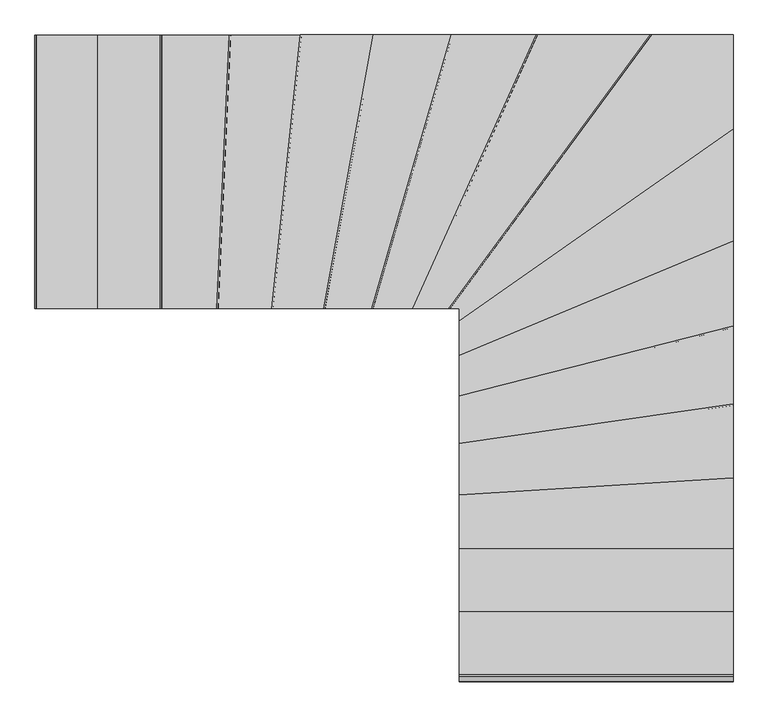
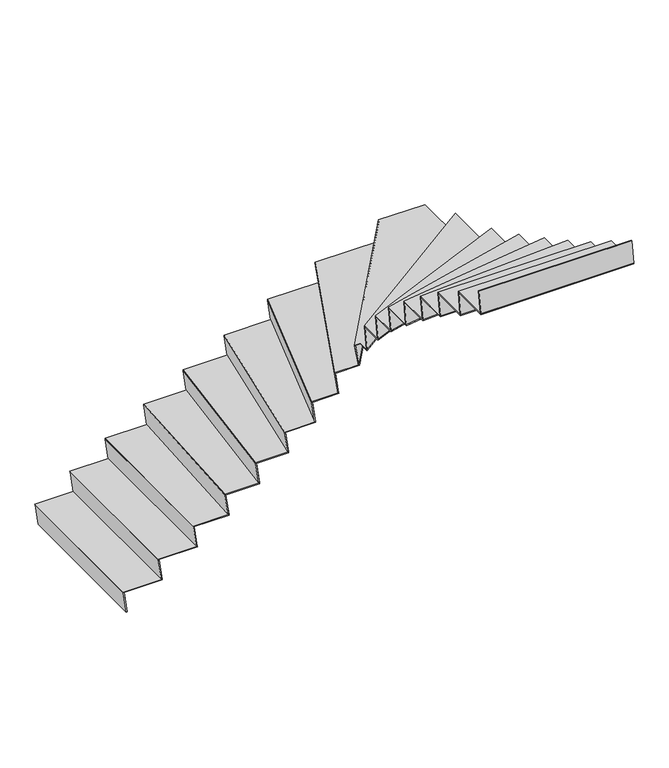
"""IFC4 building model written with IfcOpenShell, lengths in millimetres: stair flight geometry."""

import ifcopenshell
import ifcopenshell.guid

model = None  # the IFC model being written
_history = None  # IfcOwnerHistory: only IFC2X3 demands one
_inside = {}  # id of a spatial element -> (the spatial element, [elements in it])
_under = {}  # id of a project, library or spatial element -> (it, [spatial elements below it])
_declared = {}  # id of a project -> (the project, [libraries it declares])
_typed = {}  # id of a type object -> (the type object, [elements of that type])
_made_of = {}  # id of a material, layer set ... -> (it, [elements and type objects made of it])


def new_model(schema):
    """Start an empty IFC model of exactly this schema.

    Asked for "IFC4X3", IfcOpenShell would pick the latest addendum, in which some entities
    have other attributes; the version numbers below select the first issue.
    IFC2X3 requires an IfcOwnerHistory on every rooted entity: one is made here for all.
    """
    global model, _history
    if schema == "IFC4X3":
        model = ifcopenshell.file(schema_version=(4, 3, 0, 0))
    else:
        model = ifcopenshell.file(schema=schema)
    _inside.clear()
    _under.clear()
    _declared.clear()
    _typed.clear()
    _made_of.clear()
    _history = None
    if model.schema == "IFC2X3":
        org = make("IfcOrganization", Name="unknown")
        user = make(
            "IfcPersonAndOrganization",
            ThePerson=make("IfcPerson", FamilyName="unknown"),
            TheOrganization=org,
        )
        app = make(
            "IfcApplication",
            ApplicationDeveloper=org,
            Version="unknown",
            ApplicationFullName="unknown",
            ApplicationIdentifier="unknown",
        )
        _history = make(
            "IfcOwnerHistory",
            OwningUser=user,
            OwningApplication=app,
            ChangeAction="ADDED",
            CreationDate=0,
        )
    return model


def make(cls, **values):
    """One entity of the class cls with the attributes given. An attribute that is None is left unset."""
    return model.create_entity(
        cls, **{name: value for name, value in values.items() if value is not None}
    )


def rooted(cls, **values):
    """An entity with a GlobalId (a new one), such as an element, a storey or a relation."""
    return make(cls, GlobalId=ifcopenshell.guid.new(), OwnerHistory=_history, **values)


def si_unit(unit_type, name, prefix=None):
    """IfcSIUnit, for example si_unit("LENGTHUNIT", "METRE", prefix="MILLI")."""
    return make("IfcSIUnit", UnitType=unit_type, Prefix=prefix, Name=name)


def assignment(units):
    """IfcUnitAssignment: the units of a project."""
    return None if units is None else make("IfcUnitAssignment", Units=units)


def point(xyz):
    """IfcCartesianPoint."""
    return None if xyz is None else make("IfcCartesianPoint", Coordinates=xyz)


def direction(xyz):
    """IfcDirection."""
    return None if xyz is None else make("IfcDirection", DirectionRatios=xyz)


def frame(location, z_axis=None, x_axis=None):
    """IfcAxis2Placement3D, a coordinate frame: its origin and axes. An axis left out is left unset."""
    return make(
        "IfcAxis2Placement3D",
        Location=point(location),
        Axis=direction(z_axis),
        RefDirection=direction(x_axis),
    )


def origin():
    """The frame at (0, 0, 0) with its axes left unset."""
    return frame((0.0, 0.0, 0.0))


def place(relative_to, where):
    """IfcLocalPlacement: puts the frame where relative to a parent placement (None: the world)."""
    return make(
        "IfcLocalPlacement", PlacementRelTo=relative_to, RelativePlacement=where
    )


def context(
    kind, dimensions, precision=None, world=None, true_north=None, identifier=None
):
    """IfcGeometricRepresentationContext, for example the 3D "Model" context."""
    return make(
        "IfcGeometricRepresentationContext",
        ContextIdentifier=identifier,
        ContextType=kind,
        CoordinateSpaceDimension=dimensions,
        Precision=precision,
        WorldCoordinateSystem=world,
        TrueNorth=true_north,
    )


def project(units=None, contexts=None):
    """IfcProject with its units and contexts."""
    return rooted(
        "IfcProject",
        Name="project",
        RepresentationContexts=contexts,
        UnitsInContext=assignment(units),
    )


def spatial(cls, under=None, at=None, **own):
    """A site, building, storey or space (cls), placed at a placement, below another one or the project."""
    s = rooted(cls, ObjectPlacement=at, **own)
    if under is not None:
        _under.setdefault(under.id(), (under, []))[1].append(s)
    return s


def faces_of(points, faces, orient=None, outer=None):
    """IfcFace entities. A face is a list of loops; a loop is a list of indices into points, from 0.

    orient and outer hold one flag for each loop. By default every Orientation is true, the
    first loop of a face is its IfcFaceOuterBound and the others are IfcFaceBound.
    """
    made = []
    for i, loops in enumerate(faces):
        bounds = []
        for j, loop in enumerate(loops):
            is_outer = j == 0 if outer is None else outer[i][j]
            bounds.append(
                make(
                    "IfcFaceOuterBound" if is_outer else "IfcFaceBound",
                    Bound=make("IfcPolyLoop", Polygon=[points[k] for k in loop]),
                    Orientation=True if orient is None else orient[i][j],
                )
            )
        made.append(make("IfcFace", Bounds=bounds))
    return made


def faceted_brep(points, faces, orient=None, outer=None, voids=None):
    """IfcFacetedBrep: a solid bounded by flat faces; with voids (closed shells), ...WithVoids."""
    shared = [point(p) for p in points]
    hull = make("IfcClosedShell", CfsFaces=faces_of(shared, faces, orient, outer))
    if voids is None:
        return make("IfcFacetedBrep", Outer=hull)
    return make(
        "IfcFacetedBrepWithVoids",
        Outer=hull,
        Voids=[
            make(cls, CfsFaces=faces_of(shared, fs, o, b)) for cls, fs, o, b in voids
        ],
    )


def shape(context_of_items, identifier, shape_type, items):
    """IfcShapeRepresentation: the items that make up one representation, for example the "Body"."""
    return make(
        "IfcShapeRepresentation",
        ContextOfItems=context_of_items,
        RepresentationIdentifier=identifier,
        RepresentationType=shape_type,
        Items=items,
    )


def source(mapping_origin, context_of_items, identifier, shape_type, items):
    """IfcRepresentationMap: a shape defined once, which mapped items show again and again."""
    return make(
        "IfcRepresentationMap",
        MappingOrigin=mapping_origin,
        MappedRepresentation=shape(context_of_items, identifier, shape_type, items),
    )


def transform(
    local_origin,
    x_axis=None,
    y_axis=None,
    z_axis=None,
    scale=None,
    scale2=None,
    scale3=None,
    uniform=True,
):
    """IfcCartesianTransformationOperator3D, or its non-uniform kind. x_axis, y_axis, z_axis: its Axis1, 2, 3."""
    if uniform:
        return make(
            "IfcCartesianTransformationOperator3D",
            Axis1=direction(x_axis),
            Axis2=direction(y_axis),
            LocalOrigin=point(local_origin),
            Scale=scale,
            Axis3=direction(z_axis),
        )
    return make(
        "IfcCartesianTransformationOperator3DnonUniform",
        Axis1=direction(x_axis),
        Axis2=direction(y_axis),
        LocalOrigin=point(local_origin),
        Scale=scale,
        Axis3=direction(z_axis),
        Scale2=scale2,
        Scale3=scale3,
    )


def mapped(mapping_source, mapping_target):
    """IfcMappedItem: shows the shape of a source again, moved by a transform."""
    return make(
        "IfcMappedItem", MappingSource=mapping_source, MappingTarget=mapping_target
    )


def made_of(thing, what):
    """Note that an element or type object is made of a material, layer set ...; save() writes the relation."""
    if what is not None:
        _made_of.setdefault(what.id(), (what, []))[1].append(thing)
    return thing


def element(
    cls,
    number,
    at=None,
    inside=None,
    cuts=None,
    type_object=None,
    material=None,
    context=None,
    identifier="Body",
    shape_type=None,
    held_by="IfcProductDefinitionShape",
    body=None,
    shapes=None,
    **own,
):
    """One element of the class cls, such as IfcWall. Its Tag is "e" and its number.

    at: its placement. inside: the storey or other place that contains it. cuts: it is an
    opening in that element (IfcRelVoidsElement). A single representation is given by context,
    identifier, shape_type and body (its items); several are given by shapes. held_by: the class
    of the entity that holds the representations. save() writes the other relations.
    """
    e = rooted(cls, Tag="e%d" % number, ObjectPlacement=at, **own)
    if body is not None:
        shapes = [shape(context, identifier, shape_type, body)]
    if shapes is not None:
        e.Representation = make(held_by, Representations=shapes)
    if inside is not None:
        _inside.setdefault(inside.id(), (inside, []))[1].append(e)
    if cuts is not None:
        rooted(
            "IfcRelVoidsElement", RelatingBuildingElement=cuts, RelatedOpeningElement=e
        )
    if type_object is not None:
        _typed.setdefault(type_object.id(), (type_object, []))[1].append(e)
    return made_of(e, material)


def aggregate(whole, parts):
    """IfcRelAggregates: a whole, such as a stair, and the parts it consists of."""
    return rooted("IfcRelAggregates", RelatingObject=whole, RelatedObjects=parts)


def save(model, path):
    """Write the relations noted so far, then the file.

    IfcRelAggregates (storeys below a building ...), IfcRelContainedInSpatialStructure (elements
    in a storey), IfcRelDefinesByType, IfcRelAssociatesMaterial and IfcRelDeclares: one each for
    every whole, place, type object, material and project.
    """
    for whole, parts in _under.values():
        aggregate(whole, parts)
    for where, things in _inside.values():
        rooted(
            "IfcRelContainedInSpatialStructure",
            RelatedElements=things,
            RelatingStructure=where,
        )
    for kind, things in _typed.values():
        rooted("IfcRelDefinesByType", RelatedObjects=things, RelatingType=kind)
    for what, things in _made_of.values():
        rooted("IfcRelAssociatesMaterial", RelatedObjects=things, RelatingMaterial=what)
    for by, libraries in _declared.values():
        rooted("IfcRelDeclares", RelatingContext=by, RelatedDefinitions=libraries)
    model.write(path)


def stair_flight_54cb2c30(model_context):
    return source(origin(), model_context, "Body", "Brep", [
        faceted_brep([(1096.1046783, 2871.77305, 176.4705882), (1096.9546783, 2871.77305, 170.4705882), (1096.9546783, 4071.77305, 170.4705882), (1096.1046783, 4071.77305, 176.4705882), (790.0447691, 4071.77305, 176.4705882), (790.0447691, 2871.77305, 176.4705882), (790.8947691, 2871.77305, 170.4705882), (790.8947691, 4071.77305, 170.4705882)], [[[0, 1, 2, 3]], [[3, 4, 5, 0]], [[2, 1, 6, 7]], [[4, 3, 2, 7]], [[0, 5, 6, 1]], [[5, 4, 7, 6]]]),
        faceted_brep([(790.8947691, 2871.77305, 170.4705882), (815.0447691, 2871.77305, 0.0), (821.1046783, 2871.77305, 0.0), (796.9546783, 2871.77305, 170.4705882), (790.8947691, 4071.77305, 170.4705882), (796.9546783, 4071.77305, 170.4705882), (821.1046783, 4071.77305, 0.0), (815.0447691, 4071.77305, 0.0)], [[[0, 1, 2, 3]], [[4, 5, 6, 7]], [[1, 0, 4, 7]], [[2, 1, 7, 6]], [[3, 2, 6, 5]], [[0, 3, 5, 4]]]),
        faceted_brep([(1065.8947691, 2871.77305, 346.9411765), (1090.0447691, 2871.77305, 176.4705882), (1096.1046783, 2871.77305, 176.4705882), (1071.9546783, 2871.77305, 346.9411765), (1065.8947691, 4071.77305, 346.9411765), (1071.9546783, 4071.77305, 346.9411765), (1096.1046783, 4071.77305, 176.4705882), (1090.0447691, 4071.77305, 176.4705882)], [[[0, 1, 2, 3]], [[4, 5, 6, 7]], [[1, 0, 4, 7]], [[2, 1, 7, 6]], [[3, 2, 6, 5]], [[0, 3, 5, 4]]]),
        faceted_brep([(1371.1046783, 4071.77305, 352.9411765), (1065.0447691, 4071.77305, 352.9411765), (1065.0447691, 2871.77305, 352.9411765), (1371.1046783, 2871.77305, 352.9411765), (1371.9546783, 4071.77305, 346.9411765), (1371.9546783, 2871.77305, 346.9411765), (1065.8947691, 2871.77305, 346.9411765), (1065.8947691, 4071.77305, 346.9411765)], [[[0, 1, 2, 3]], [[4, 5, 6, 7]], [[1, 0, 4, 7]], [[3, 2, 6, 5]], [[3, 5, 4, 0]], [[2, 1, 7, 6]]]),
        faceted_brep([(1340.8947691, 2871.77305, 523.4117647), (1365.0447691, 2871.77305, 352.9411765), (1371.1046783, 2871.77305, 352.9411765), (1346.9546783, 2871.77305, 523.4117647), (1340.8947691, 4071.77305, 523.4117647), (1346.9546783, 4071.77305, 523.4117647), (1371.1046783, 4071.77305, 352.9411765), (1365.0447691, 4071.77305, 352.9411765)], [[[0, 1, 2, 3]], [[4, 5, 6, 7]], [[1, 0, 4, 7]], [[2, 1, 7, 6]], [[3, 2, 6, 5]], [[0, 3, 5, 4]]]),
        faceted_brep([(1673.5053782, 4071.77305, 529.4117647), (1340.0447691, 4071.77305, 529.4117647), (1340.0447691, 2871.77305, 529.4117647), (1618.7685693, 2871.77305, 529.4117647), (1674.356262, 4071.77305, 523.4117647), (1619.6194531, 2871.77305, 523.4117647), (1340.8947691, 2871.77305, 523.4117647), (1340.8947691, 4071.77305, 523.4117647)], [[[0, 1, 2, 3]], [[4, 5, 6, 7]], [[1, 0, 4, 7]], [[3, 2, 6, 5]], [[3, 5, 4, 0]], [[2, 1, 7, 6]]]),
        faceted_brep([(1588.5272484, 2871.77305, 699.8823529), (1612.7023591, 2871.77305, 529.4117647), (1618.7685693, 2871.77305, 529.4117647), (1594.5934586, 2871.77305, 699.8823529), (1643.2640574, 4071.77305, 699.8823529), (1649.3302676, 4071.77305, 699.8823529), (1673.5053782, 4071.77305, 529.4117647), (1667.439168, 4071.77305, 529.4117647)], [[[0, 1, 2, 3]], [[4, 5, 6, 7]], [[1, 0, 4, 7]], [[2, 1, 7, 6]], [[3, 2, 6, 5]], [[0, 3, 5, 4]]]),
        faceted_brep([(1983.6993098, 4071.77305, 705.8823529), (1642.4131736, 4071.77305, 705.8823529), (1587.6763646, 2871.77305, 705.8823529), (1858.8453761, 2871.77305, 705.8823529), (1984.5538982, 4071.77305, 699.8823529), (1859.6999645, 2871.77305, 699.8823529), (1588.5272484, 2871.77305, 699.8823529), (1643.2640574, 4071.77305, 699.8823529)], [[[0, 1, 2, 3]], [[4, 5, 6, 7]], [[1, 0, 4, 7]], [[3, 2, 6, 5]], [[3, 5, 4, 0]], [[2, 1, 7, 6]]]),
        faceted_brep([(1828.4723906, 2871.77305, 876.3529412), (1852.7527549, 2871.77305, 705.8823529), (1858.8453761, 2871.77305, 705.8823529), (1834.5650119, 2871.77305, 876.3529412), (1953.3263243, 4071.77305, 876.3529412), (1959.4189456, 4071.77305, 876.3529412), (1983.6993098, 4071.77305, 705.8823529), (1977.6066886, 4071.77305, 705.8823529)], [[[0, 1, 2, 3]], [[4, 5, 6, 7]], [[1, 0, 4, 7]], [[2, 1, 7, 6]], [[3, 2, 6, 5]], [[0, 3, 5, 4]]]),
        faceted_brep([(2305.5593008, 4071.77305, 882.3529412), (1952.4717359, 4071.77305, 882.3529412), (1827.6178022, 2871.77305, 882.3529412), (2087.6658131, 2871.77305, 882.3529412), (2306.4231996, 4071.77305, 876.3529412), (2088.529712, 2871.77305, 876.3529412), (1828.4723906, 2871.77305, 876.3529412), (1953.3263243, 4071.77305, 876.3529412)], [[[0, 1, 2, 3]], [[4, 5, 6, 7]], [[1, 0, 4, 7]], [[3, 2, 6, 5]], [[3, 5, 4, 0]], [[2, 1, 7, 6]]]),
        faceted_brep([(2056.9619241, 2871.77305, 1052.8235294), (2081.5068148, 2871.77305, 882.3529412), (2087.6658131, 2871.77305, 882.3529412), (2063.1209225, 2871.77305, 1052.8235294), (2274.8554117, 4071.77305, 1052.8235294), (2281.0144101, 4071.77305, 1052.8235294), (2305.5593008, 4071.77305, 882.3529412), (2299.4003024, 4071.77305, 882.3529412)], [[[0, 1, 2, 3]], [[4, 5, 6, 7]], [[1, 0, 4, 7]], [[2, 1, 7, 6]], [[3, 2, 6, 5]], [[0, 3, 5, 4]]]),
        faceted_brep([(2646.0254998, 4071.77305, 1058.8235294), (2273.9915129, 4071.77305, 1058.8235294), (2056.0980253, 2871.77305, 1058.8235294), (2298.7330773, 2871.77305, 1058.8235294), (2646.9103814, 4071.77305, 1052.8235294), (2299.6179589, 2871.77305, 1052.8235294), (2056.9619241, 2871.77305, 1052.8235294), (2274.8554117, 4071.77305, 1052.8235294)], [[[0, 1, 2, 3]], [[4, 5, 6, 7]], [[1, 0, 4, 7]], [[3, 2, 6, 5]], [[3, 5, 4, 0]], [[2, 1, 7, 6]]]),
        faceted_brep([(2267.2834394, 2871.77305, 1229.2941176), (2292.4244867, 2871.77305, 1058.8235294), (2298.7330773, 2871.77305, 1058.8235294), (2273.5920301, 2871.77305, 1229.2941176), (2614.5758619, 4071.77305, 1229.2941176), (2620.8844526, 4071.77305, 1229.2941176), (2646.0254998, 4071.77305, 1058.8235294), (2639.7169091, 4071.77305, 1058.8235294)], [[[0, 1, 2, 3]], [[4, 5, 6, 7]], [[1, 0, 4, 7]], [[2, 1, 7, 6]], [[3, 2, 6, 5]], [[0, 3, 5, 4]]]),
        faceted_brep([(3020.7519354, 4071.77305, 1235.2941176), (2613.6909803, 4071.77305, 1235.2941176), (2266.3985579, 2871.77305, 1235.2941176), (2480.5963819, 2871.77305, 1235.2941176), (3021.6840784, 4071.77305, 1229.2941176), (2481.5285249, 2871.77305, 1229.2941176), (2267.2834394, 2871.77305, 1229.2941176), (2614.5758619, 4071.77305, 1229.2941176)], [[[0, 1, 2, 3]], [[4, 5, 6, 7]], [[1, 0, 4, 7]], [[3, 2, 6, 5]], [[3, 5, 4, 0]], [[2, 1, 7, 6]]]),
        faceted_brep([(2447.467023, 2871.77305, 1405.7647059), (2473.9508503, 2871.77305, 1235.2941176), (2480.5963819, 2871.77305, 1235.2941176), (2454.1125547, 2871.77305, 1405.7647059), (2987.6225764, 4071.77305, 1405.7647059), (2994.2681081, 4071.77305, 1405.7647059), (3020.7519354, 4071.77305, 1235.2941176), (3014.1064037, 4071.77305, 1235.2941176)], [[[0, 1, 2, 3]], [[4, 5, 6, 7]], [[1, 0, 4, 7]], [[2, 1, 7, 6]], [[3, 2, 6, 5]], [[0, 3, 5, 4]]]),
        faceted_brep([(3524.5617135, 4071.77305, 1411.7647059), (2986.6904335, 4071.77305, 1411.7647059), (2446.53488, 2871.77305, 1411.7647059), (2641.2988686, 2871.77305, 1411.7647059), (3525.6171429, 4071.77305, 1405.7647059), (2642.3542979, 2871.77305, 1405.7647059), (2447.467023, 2871.77305, 1405.7647059), (2987.6225764, 4071.77305, 1405.7647059)], [[[0, 1, 2, 3]], [[4, 5, 6, 7]], [[1, 0, 4, 7]], [[3, 2, 6, 5]], [[3, 5, 4, 0]], [[2, 1, 7, 6]]]),
        faceted_brep([(2603.7877814, 2871.77305, 1582.2352941), (2633.774391, 2871.77305, 1411.7647059), (2641.2988686, 2871.77305, 1411.7647059), (2611.3122589, 2871.77305, 1582.2352941), (3487.0506263, 4071.77305, 1582.2352941), (3494.5751039, 4071.77305, 1582.2352941), (3524.5617135, 4071.77305, 1411.7647059), (3517.037236, 4071.77305, 1411.7647059)], [[[0, 1, 2, 3]], [[4, 5, 6, 7]], [[1, 0, 4, 7]], [[2, 1, 7, 6]], [[3, 2, 6, 5]], [[0, 3, 5, 4]]]),
        faceted_brep([(3850.0, 3620.9311691, 1588.2352941), (3850.0, 4071.77305, 1588.2352941), (3485.995197, 4071.77305, 1588.2352941), (2602.732352, 2871.77305, 1588.2352941), (2650.0, 2871.77305, 1588.2352941), (2650.0, 2779.5269645, 1588.2352941), (3850.0, 3619.8930411, 1582.2352941), (2650.0, 2778.4888366, 1582.2352941), (2650.0, 2871.77305, 1582.2352941), (2603.7877814, 2871.77305, 1582.2352941), (3487.0506263, 4071.77305, 1582.2352941), (3850.0, 4071.77305, 1582.2352941)], [[[0, 1, 2, 3, 4, 5]], [[6, 7, 8, 9, 10, 11]], [[1, 0, 6, 11]], [[2, 1, 11, 10]], [[4, 3, 9, 8]], [[5, 4, 8, 7]], [[5, 7, 6, 0]], [[3, 2, 10, 9]]]),
        faceted_brep([(2650.0, 2816.4231419, 1758.7058824), (2650.0, 2786.9280952, 1588.2352941), (2650.0, 2779.5269645, 1588.2352941), (2650.0, 2809.0220112, 1758.7058824), (3850.0, 3657.8273465, 1758.7058824), (3850.0, 3650.4262158, 1758.7058824), (3850.0, 3620.9311691, 1588.2352941), (3850.0, 3628.3322998, 1588.2352941)], [[[0, 1, 2, 3]], [[4, 5, 6, 7]], [[1, 0, 4, 7]], [[2, 1, 7, 6]], [[3, 2, 6, 5]], [[0, 3, 5, 4]]]),
        faceted_brep([(3850.0, 3134.7334972, 1764.7058824), (3850.0, 3658.8654744, 1764.7058824), (2650.0, 2817.4612699, 1764.7058824), (2650.0, 2632.6587702, 1764.7058824), (3850.0, 3133.8120976, 1758.7058824), (2650.0, 2631.7373707, 1758.7058824), (2650.0, 2816.4231419, 1758.7058824), (3850.0, 3657.8273465, 1758.7058824)], [[[0, 1, 2, 3]], [[4, 5, 6, 7]], [[1, 0, 4, 7]], [[3, 2, 6, 5]], [[3, 5, 4, 0]], [[2, 1, 7, 6]]]),
        faceted_brep([(2650.0, 2665.4062963, 1935.1764706), (2650.0, 2639.2277087, 1764.7058824), (2650.0, 2632.6587702, 1764.7058824), (2650.0, 2658.8373578, 1935.1764706), (3850.0, 3167.4810232, 1935.1764706), (3850.0, 3160.9120847, 1935.1764706), (3850.0, 3134.7334972, 1764.7058824), (3850.0, 3141.3024357, 1764.7058824)], [[[0, 1, 2, 3]], [[4, 5, 6, 7]], [[1, 0, 4, 7]], [[2, 1, 7, 6]], [[3, 2, 6, 5]], [[0, 3, 5, 4]]]),
        faceted_brep([(3850.0, 2762.6639562, 1941.1764706), (3850.0, 3168.4024228, 1941.1764706), (2650.0, 2666.3276958, 1941.1764706), (2650.0, 2456.5603699, 1941.1764706), (3850.0, 2761.7867376, 1935.1764706), (2650.0, 2455.6831513, 1935.1764706), (2650.0, 2665.4062963, 1935.1764706), (3850.0, 3167.4810232, 1935.1764706)], [[[0, 1, 2, 3]], [[4, 5, 6, 7]], [[1, 0, 4, 7]], [[3, 2, 6, 5]], [[3, 5, 4, 0]], [[2, 1, 7, 6]]]),
        faceted_brep([(2650.0, 2487.7376553, 2111.6470588), (2650.0, 2462.8143284, 1941.1764706), (2650.0, 2456.5603699, 1941.1764706), (2650.0, 2481.4836968, 2111.6470588), (3850.0, 2793.8412416, 2111.6470588), (3850.0, 2787.587283, 2111.6470588), (3850.0, 2762.6639562, 1941.1764706), (3850.0, 2768.9179147, 1941.1764706)], [[[0, 1, 2, 3]], [[4, 5, 6, 7]], [[1, 0, 4, 7]], [[2, 1, 7, 6]], [[3, 2, 6, 5]], [[0, 3, 5, 4]]]),
        faceted_brep([(3850.0, 2421.2797748, 2117.6470588), (3850.0, 2794.7184601, 2117.6470588), (2650.0, 2488.6148739, 2117.6470588), (2650.0, 2249.2990176, 2117.6470588), (3850.0, 2420.4210897, 2111.6470588), (2650.0, 2248.4403326, 2111.6470588), (2650.0, 2487.7376553, 2111.6470588), (3850.0, 2793.8412416, 2111.6470588)], [[[0, 1, 2, 3]], [[4, 5, 6, 7]], [[1, 0, 4, 7]], [[3, 2, 6, 5]], [[3, 5, 4, 0]], [[2, 1, 7, 6]]]),
        faceted_brep([(2650.0, 2279.8176034, 2288.1176471), (2650.0, 2255.4208454, 2117.6470588), (2650.0, 2249.2990176, 2117.6470588), (2650.0, 2273.6957757, 2288.1176471), (3850.0, 2451.7983605, 2288.1176471), (3850.0, 2445.6765328, 2288.1176471), (3850.0, 2421.2797748, 2117.6470588), (3850.0, 2427.4016025, 2117.6470588)], [[[0, 1, 2, 3]], [[4, 5, 6, 7]], [[1, 0, 4, 7]], [[2, 1, 7, 6]], [[3, 2, 6, 5]], [[0, 3, 5, 4]]]),
        faceted_brep([(3850.0, 2097.7004095, 2294.1176471), (3850.0, 2452.6570456, 2294.1176471), (2650.0, 2280.6762884, 2294.1176471), (2650.0, 2023.3941263, 2294.1176471), (3850.0, 2096.8487814, 2288.1176471), (2650.0, 2022.5424983, 2288.1176471), (2650.0, 2279.8176034, 2288.1176471), (3850.0, 2451.7983605, 2288.1176471)], [[[0, 1, 2, 3]], [[4, 5, 6, 7]], [[1, 0, 4, 7]], [[3, 2, 6, 5]], [[3, 5, 4, 0]], [[2, 1, 7, 6]]]),
        faceted_brep([(2650.0, 2053.6618974, 2464.5882353), (2650.0, 2029.4656422, 2294.1176471), (2650.0, 2023.3941263, 2294.1176471), (2650.0, 2047.5903814, 2464.5882353), (3850.0, 2127.9681806, 2464.5882353), (3850.0, 2121.8966646, 2464.5882353), (3850.0, 2097.7004095, 2294.1176471), (3850.0, 2103.7719254, 2294.1176471)], [[[0, 1, 2, 3]], [[4, 5, 6, 7]], [[1, 0, 4, 7]], [[2, 1, 7, 6]], [[3, 2, 6, 5]], [[0, 3, 5, 4]]]),
        faceted_brep([(3850.0, 1785.6067578, 2470.5882353), (3850.0, 2128.8198086, 2470.5882353), (2650.0, 2054.5135254, 2470.5882353), (2650.0, 1785.6067578, 2470.5882353), (3850.0, 1784.7567578, 2464.5882353), (2650.0, 1784.7567578, 2464.5882353), (2650.0, 2053.6618974, 2464.5882353), (3850.0, 2127.9681806, 2464.5882353)], [[[0, 1, 2, 3]], [[4, 5, 6, 7]], [[1, 0, 4, 7]], [[3, 2, 6, 5]], [[3, 5, 4, 0]], [[2, 1, 7, 6]]]),
        faceted_brep([(2650.0, 1815.816667, 2641.0588235), (2650.0, 1791.666667, 2470.5882353), (2650.0, 1785.6067578, 2470.5882353), (2650.0, 1809.7567578, 2641.0588235), (3850.0, 1815.816667, 2641.0588235), (3850.0, 1809.7567578, 2641.0588235), (3850.0, 1785.6067578, 2470.5882353), (3850.0, 1791.666667, 2470.5882353)], [[[0, 1, 2, 3]], [[4, 5, 6, 7]], [[1, 0, 4, 7]], [[2, 1, 7, 6]], [[3, 2, 6, 5]], [[0, 3, 5, 4]]]),
        faceted_brep([(3850.0, 1510.6067578, 2647.0588235), (3850.0, 1816.666667, 2647.0588235), (2650.0, 1816.666667, 2647.0588235), (2650.0, 1510.6067578, 2647.0588235), (3850.0, 1509.7567578, 2641.0588235), (2650.0, 1509.7567578, 2641.0588235), (2650.0, 1815.816667, 2641.0588235), (3850.0, 1815.816667, 2641.0588235)], [[[0, 1, 2, 3]], [[4, 5, 6, 7]], [[1, 0, 4, 7]], [[3, 2, 6, 5]], [[3, 5, 4, 0]], [[2, 1, 7, 6]]]),
        faceted_brep([(2650.0, 1540.816667, 2817.5294118), (2650.0, 1516.666667, 2647.0588235), (2650.0, 1510.6067578, 2647.0588235), (2650.0, 1534.7567578, 2817.5294118), (3850.0, 1540.816667, 2817.5294118), (3850.0, 1534.7567578, 2817.5294118), (3850.0, 1510.6067578, 2647.0588235), (3850.0, 1516.666667, 2647.0588235)], [[[0, 1, 2, 3]], [[4, 5, 6, 7]], [[1, 0, 4, 7]], [[2, 1, 7, 6]], [[3, 2, 6, 5]], [[0, 3, 5, 4]]]),
        faceted_brep([(2650.0, 1265.816667, 2994.0), (2650.0, 1241.666667, 2823.5294118), (2650.0, 1235.6067578, 2823.5294118), (2650.0, 1259.7567578, 2994.0), (3850.0, 1265.816667, 2994.0), (3850.0, 1259.7567578, 2994.0), (3850.0, 1235.6067578, 2823.5294118), (3850.0, 1241.666667, 2823.5294118)], [[[0, 1, 2, 3]], [[4, 5, 6, 7]], [[1, 0, 4, 7]], [[2, 1, 7, 6]], [[3, 2, 6, 5]], [[0, 3, 5, 4]]]),
        faceted_brep([(3850.0, 1235.6067578, 2823.5294118), (3850.0, 1541.666667, 2823.5294118), (2650.0, 1541.666667, 2823.5294118), (2650.0, 1235.6067578, 2823.5294118), (3850.0, 1234.7567578, 2817.5294118), (2650.0, 1234.7567578, 2817.5294118), (2650.0, 1540.816667, 2817.5294118), (3850.0, 1540.816667, 2817.5294118)], [[[0, 1, 2, 3]], [[4, 5, 6, 7]], [[1, 0, 4, 7]], [[3, 2, 6, 5]], [[3, 5, 4, 0]], [[2, 1, 7, 6]]]),
    ])


if __name__ == "__main__":
    model = new_model("IFC4")
    model_context = context("Model", 3, world=origin())
    ifc_project = project(units=[si_unit("LENGTHUNIT", "METRE", prefix="MILLI")], contexts=[model_context])
    site = spatial("IfcSite", under=ifc_project)
    building = spatial("IfcBuilding", under=site)
    placement = place(None, origin())
    stair_flight_shape = stair_flight_54cb2c30(model_context)
    element("IfcStairFlight", 1, at=placement, inside=building, context=model_context, shape_type="MappedRepresentation", body=[
        mapped(stair_flight_shape, transform((0.0, 0.0, 0.0), x_axis=(1.0, 0.0, 0.0), y_axis=(0.0, 1.0, 0.0), z_axis=(0.0, 0.0, 1.0))),
    ])
    save(model, "model.ifc")

# Revit data of these elements
# Element 1 (IfcStairFlight)
#   Materials on its faces: "Acero, acabado de pintura, gris oscuro"
# Materials
#   "Acero, acabado de pintura, gris oscuro": class "Metal", colour RGB 89 89 89, transparency 0, Description = "Acero, acabado de pintura, gris oscuro, brillante", Cost = 0
